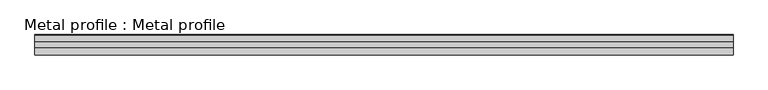
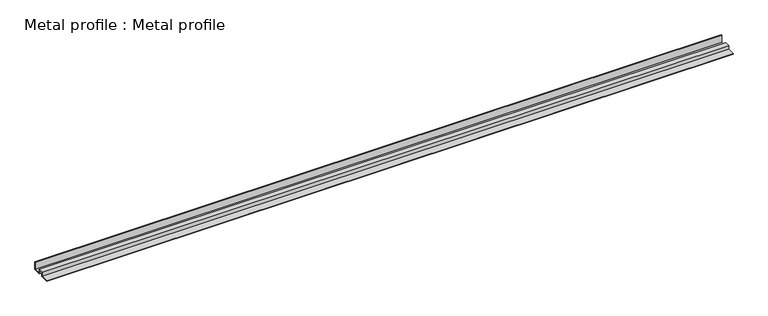
"""IFC4 building model written with IfcOpenShell, lengths in millimetres: proxy geometry, Metal profile : Metal profile."""

from ifc_helpers import new_model, si_unit, frame, origin, place, context, project, spatial, polyline, outline, extrude, source, transform, mapped, element, save


def metal_profile_metal_profile_1631b574(model_context):
    return source(origin(), model_context, "Body", "SweptSolid", [
        extrude(outline(polyline([(10462.1750834, 39401.496), (10439.9500834, 39401.496), (10439.9500834, 39412.926), (10427.2500834, 39412.926), (10427.2500834, 39401.496), (10403.5368994, 39401.496), (10403.5368994, 39402.776), (10425.9700834, 39402.776), (10425.9700834, 39414.206), (10441.2300834, 39414.206), (10441.2300834, 39402.776), (10460.8950834, 39402.776), (10460.8950834, 39425.2967615), (10462.1750834, 39425.2967615), (10462.1750834, 39401.496)])), frame((3694.2883192, 0.0, 0.0), z_axis=(1.0, 0.0, 0.0), x_axis=(0.0, 1.0, 0.0)), (0.0, 0.0, 1.0), 2000.0),
    ])


if __name__ == "__main__":
    model = new_model("IFC4")
    model_context = context("Model", 3, world=origin())
    ifc_project = project(units=[si_unit("LENGTHUNIT", "METRE", prefix="MILLI")], contexts=[model_context])
    site = spatial("IfcSite", under=ifc_project)
    building = spatial("IfcBuilding", under=site)
    placement = place(None, origin())
    metal_profile_metal_profile_shape = metal_profile_metal_profile_1631b574(model_context)
    element("IfcBuildingElementProxy", 1, Name="Metal profile : Metal profile", ObjectType="Metal profile : Metal profile", at=placement, inside=building, context=model_context, shape_type="MappedRepresentation", body=[
        mapped(metal_profile_metal_profile_shape, transform((0.0, 0.0, 0.0), x_axis=(1.0, 0.0, 0.0), y_axis=(0.0, 1.0, 0.0), z_axis=(0.0, 0.0, 1.0))),
    ])
    save(model, "model.ifc")

# Revit data of these elements
# Type "Metal profile : Metal profile"
#   NameOverride = "Metal profile"
# Element 1 (IfcBuildingElementProxy, "Metal profile : Metal profile")
#   Materials on its faces: "16 GA. COPPER SOFFIT DRIP SCREED"
# Materials
#   "16 GA. COPPER SOFFIT DRIP SCREED": class "Unassigned", colour RGB 255 217 0, transparency 0
